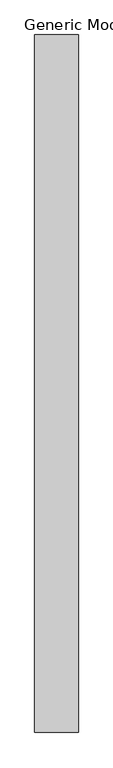
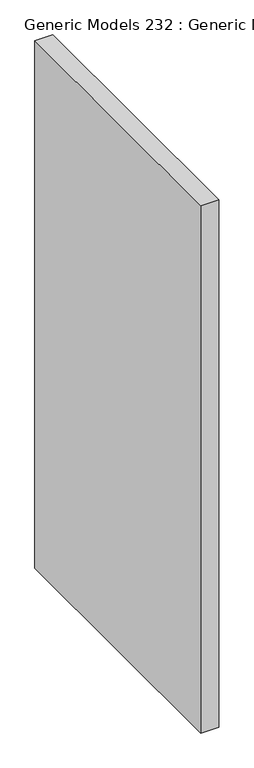
"""IFC4 building model written with IfcOpenShell, lengths in millimetres: proxy geometry, Generic Models 232 : Generic Models 1."""

from ifc_helpers import new_model, si_unit, frame, origin, place, context, project, spatial, polyline, outline, extrude, source, transform, mapped, element, save


def generic_models_232_generic_models_1_b4b06e59(model_context):
    return source(origin(), model_context, "Body", "SweptSolid", [
        extrude(outline(polyline([(49777.65, 1219.2), (49777.65, 0.0), (49701.45, 0.0), (49701.45, 1219.2), (49777.65, 1219.2)])), frame((0.0, 0.0, 3090.8625), z_axis=(0.0, 0.0, 1.0), x_axis=(1.0, 0.0, 0.0)), (0.0, 0.0, 1.0), 2368.55),
    ])


if __name__ == "__main__":
    model = new_model("IFC4")
    model_context = context("Model", 3, world=origin())
    ifc_project = project(units=[si_unit("LENGTHUNIT", "METRE", prefix="MILLI")], contexts=[model_context])
    site = spatial("IfcSite", under=ifc_project)
    building = spatial("IfcBuilding", under=site)
    placement = place(None, origin())
    generic_models_232_generic_models_1_shape = generic_models_232_generic_models_1_b4b06e59(model_context)
    element("IfcBuildingElementProxy", 1, Name="Generic Models 232 : Generic Models 1", ObjectType="Generic Models 232 : Generic Models 1", at=placement, inside=building, context=model_context, shape_type="MappedRepresentation", body=[
        mapped(generic_models_232_generic_models_1_shape, transform((0.0, 0.0, 0.0), x_axis=(1.0, 0.0, 0.0), y_axis=(0.0, 1.0, 0.0), z_axis=(0.0, 0.0, 1.0))),
    ])
    save(model, "model.ifc")

# Revit data of these elements
# Element 1 (IfcBuildingElementProxy, "Generic Models 232 : Generic Models 1")
#   Materials on its faces: "(S) SOUND BATT. INSULATION (THICKNESS TO MATCH WALL DEPTH)"
# Materials
#   "(S) SOUND BATT. INSULATION (THICKNESS TO MATCH WALL DEPTH)": class "Unassigned", colour RGB 255 255 255, transparency 0, Cost = 0
